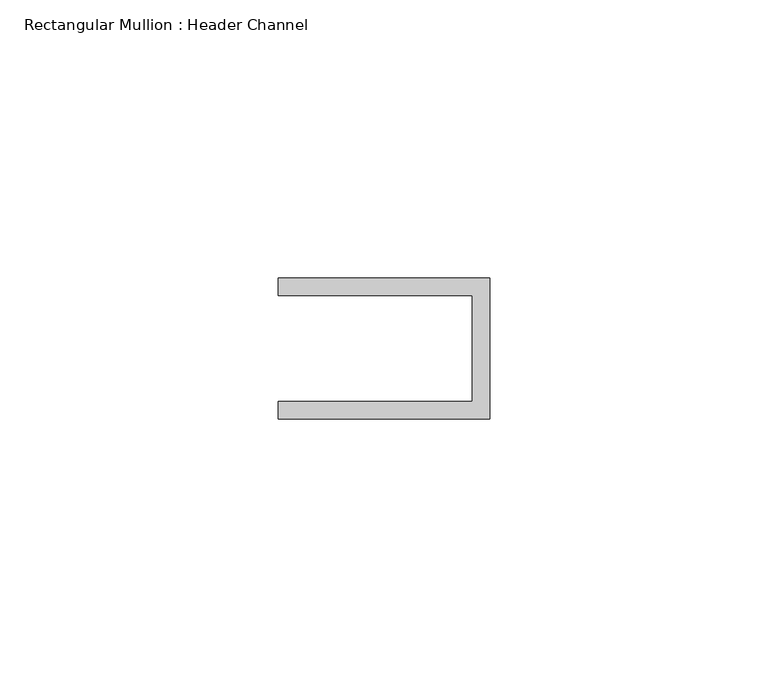
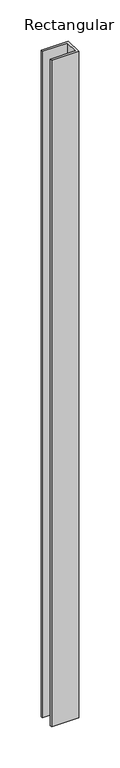
"""IFC4 building model written with IfcOpenShell, lengths in millimetres: member geometry, Rectangular Mullion : Header Channel."""

from ifc_helpers import new_model, si_unit, frame, origin, place, context, project, spatial, polyline, outline, extrude, source, transform, mapped, element, save


def rectangular_mullion_header_channel_35059403(model_context):
    return source(origin(), model_context, "Body", "SweptSolid", [
        extrude(outline(polyline([(0.0, 12.7), (0.0, -12.7), (-38.1, -12.7), (-38.1, -9.525), (-3.175, -9.525), (-3.175, 9.525), (-38.1, 9.525), (-38.1, 12.7), (0.0, 12.7)])), frame((0.0, 0.0, -990.6), z_axis=(0.0, 0.0, 1.0), x_axis=(1.0, 0.0, 0.0)), (0.0, 0.0, 1.0), 990.6),
    ])


if __name__ == "__main__":
    model = new_model("IFC4")
    model_context = context("Model", 3, world=origin())
    ifc_project = project(units=[si_unit("LENGTHUNIT", "METRE", prefix="MILLI")], contexts=[model_context])
    site = spatial("IfcSite", under=ifc_project)
    building = spatial("IfcBuilding", under=site)
    placement = place(None, origin())
    rectangular_mullion_header_channel_shape = rectangular_mullion_header_channel_35059403(model_context)
    element("IfcMember", 1, ObjectType="Rectangular Mullion : Header Channel", at=placement, inside=building, context=model_context, shape_type="MappedRepresentation", body=[
        mapped(rectangular_mullion_header_channel_shape, transform((0.0, 0.0, 0.0), x_axis=(1.0, 0.0, 0.0), y_axis=(0.0, 1.0, 0.0), z_axis=(0.0, 0.0, 1.0))),
    ])
    save(model, "model.ifc")

# Revit data of these elements
# Type "Rectangular Mullion : Header Channel"
#   built-in parameter 1007322 = 0.0833333 (stored number, unit not read)
#   built-in parameter 1007321 = -0.03125 (stored number, unit not read)
#   built-in parameter 1007320 = 0.0416667 (stored number, unit not read)
# Element 1 (IfcMember, "Rectangular Mullion : Header Channel")
#   Materials on its faces: "ALUM"
# Materials
#   "ALUM": class "Generic", colour RGB 157 157 157, transparency 0, Cost = 0
